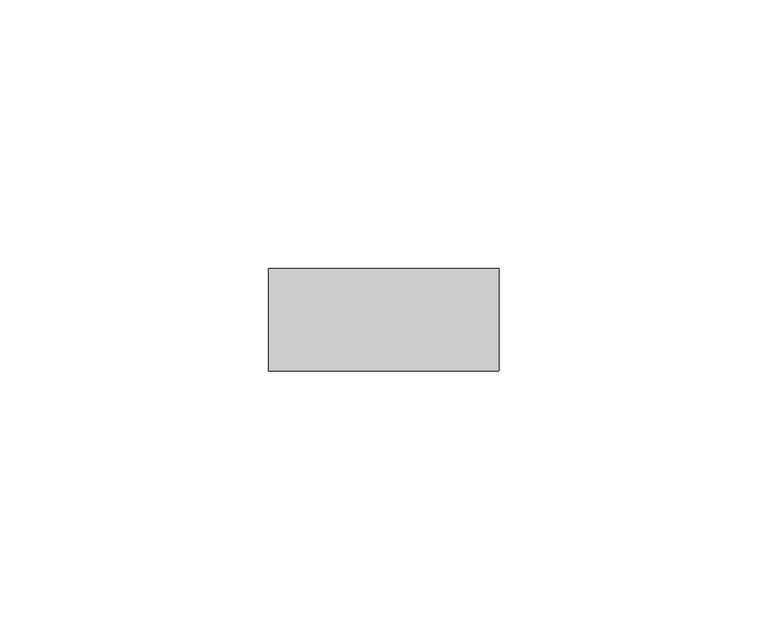
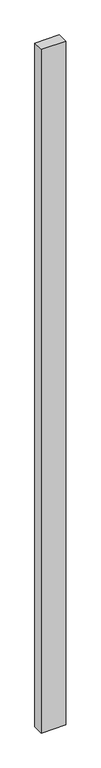
"""IFC4 building model written with IfcOpenShell, lengths in millimetres: proxy geometry, Inner panel:Inner panel:1:Inner panel:1 : Inner panel:Inner panel:300324:300043:Inner panel:1:Inner panel:1 : Inner panel:Inner panel:300324:300043 : Inner panel:Inner panel:1:Inner panel:1 : Inner panel:Inner panel:300324:300043:46 : Inner panel:Inner panel:1:Inner panel:1 : Inner panel:Inner panel:300324:300043:Inner panel:1:Inner panel:1 : Inner panel:Inner panel:300324:300043 : Inner panel:Inner panel:1:Inner panel:1 : Inner panel:Inner panel:300324:300043:300031."""

from ifc_helpers import new_model, si_unit, frame, origin, place, context, project, spatial, polyline, outline, extrude, source, transform, mapped, element, save


def generic_models_34757d3e(model_context):
    return source(origin(), model_context, "Body", "SweptSolid", [
        extrude(outline(polyline([(667523.4992239, -568253.3163841), (667566.3617239, -568253.3163841), (667566.3617239, -568272.3663841), (667523.4992239, -568272.3663841), (667523.4992239, -568253.3163841)])), frame((0.0, 0.0, 4903.3906249), z_axis=(0.0, 0.0, 1.0), x_axis=(1.0, 0.0, 0.0)), (0.0, 0.0, 1.0), 1262.4593751),
    ])


if __name__ == "__main__":
    model = new_model("IFC4")
    model_context = context("Model", 3, world=origin())
    ifc_project = project(units=[si_unit("LENGTHUNIT", "METRE", prefix="MILLI")], contexts=[model_context])
    site = spatial("IfcSite", under=ifc_project)
    building = spatial("IfcBuilding", under=site)
    placement = place(None, origin())
    generic_models_shape = generic_models_34757d3e(model_context)
    element("IfcBuildingElementProxy", 1, Name="Inner panel:Inner panel:1:Inner panel:1 : Inner panel:Inner panel:300324:300043:Inner panel:1:Inner panel:1 : Inner panel:Inner panel:300324:300043 : Inner panel:Inner panel:1:Inner panel:1 : Inner panel:Inner panel:300324:300043:46 : Inner panel:Inner panel:1:Inner panel:1 : Inner panel:Inner panel:300324:300043:Inner panel:1:Inner panel:1 : Inner panel:Inner panel:300324:300043 : Inner panel:Inner panel:1:Inner panel:1 : Inner panel:Inner panel:300324:300043:300031", ObjectType="Inner panel:Inner panel:1:Inner panel:1 : Inner panel:Inner panel:300324:300043:Inner panel:1:Inner panel:1 : Inner panel:Inner panel:300324:300043 : Inner panel:Inner panel:1:Inner panel:1 : Inner panel:Inner panel:300324:300043:46 : Inner panel:Inner panel:1:Inner panel:1 : Inner panel:Inner panel:300324:300043:Inner panel:1:Inner panel:1 : Inner panel:Inner panel:300324:300043 : Inner panel:Inner panel:1:Inner panel:1 : Inner panel:Inner panel:300324:300043:300031", at=placement, inside=building, context=model_context, shape_type="MappedRepresentation", body=[
        mapped(generic_models_shape, transform((0.0, 0.0, 0.0), x_axis=(1.0, 0.0, 0.0), y_axis=(0.0, 1.0, 0.0), z_axis=(0.0, 0.0, 1.0))),
    ])
    save(model, "model.ifc")

# Revit data of these elements
# Type "Inner panel:Inner panel:1:Inner panel:1 : Inner panel:Inner panel:300324:300043:Inner panel:1:Inner panel:1 : Inner panel:Inner panel:300324:300043 : Inner panel:Inner panel:1:Inner panel:1 : Inner panel:Inner panel:300324:300043:46 : Inner panel:Inner panel:1:Inner panel:1 : Inner panel:Inner panel:300324:300043:Inner panel:1:Inner panel:1 : Inner panel:Inner panel:300324:300043 : Inner panel:Inner panel:1:Inner panel:1 : Inner panel:Inner panel:300324:300043:300031"
#   NameOverride = "Inner panel:Inner panel:1:Inner panel:1 : Inner panel:Inner panel:300324:300043:Inner panel:1:Inner panel:1 : Inner panel:Inner panel:300324:300043 : Inner panel:Inner panel:1:Inner panel:1 : Inner panel:Inner panel:300324:300043:300031"
#   ObjectTypeOverride = "Inner panel:1:Inner panel:1 : Inner panel:Inner panel:300324:300043 : Inner panel:Inner panel:1:Inner panel:1 : Inner panel:Inner panel:300324:300043"
#   Reference = "Inner panel"
#   Tag = "300031"
# Element 1 (IfcBuildingElementProxy, "Inner panel:Inner panel:1:Inner panel:1 : Inner panel:Inner panel:300324:300043:Inner panel:1:Inner panel:1 : Inner panel:Inner panel:300324:300043 : Inner panel:Inner panel:1:Inner panel:1 : Inner panel:Inner panel:300324:300043:46 : Inner panel:Inner panel:1:Inner panel:1 : Inner panel:Inner panel:300324:300043:Inner panel:1:Inner panel:1 : Inner panel:Inner panel:300324:300043 : Inner panel:Inner panel:1:Inner panel:1 : Inner panel:Inner panel:300324:300043:300031")
#   Materials on its faces: "3/4\" EXTERIOR GRADE FIRE RETARDANT PLYWOOD (FINISH: GRADE B)"
# Materials
#   "3/4\" EXTERIOR GRADE FIRE RETARDANT PLYWOOD (FINISH: GRADE B)": class "Wood", colour RGB 149 120 74, transparency 0, Description = "Plywood, sheathing grade", Cost = 0
